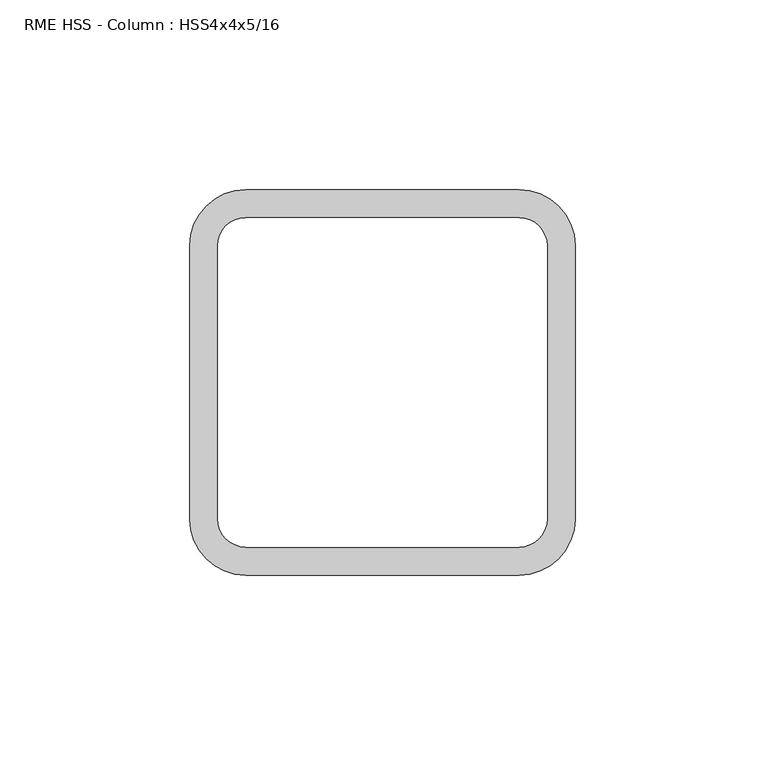
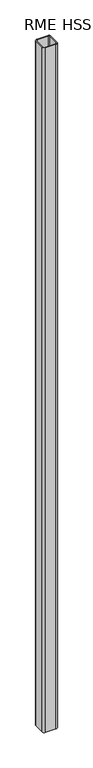
"""IFC4 building model written with IfcOpenShell, lengths in millimetres: column geometry, RME HSS - Column : HSS4x4x5/16."""

from ifc_helpers import new_model, si_unit, point, frame, frame_2d, origin, place, context, project, spatial, polyline, circle_curve, trimmed, segment, composite_curve, outline, extrude, source, transform, mapped, element, save


def rme_hss_column_hss4x4x5_16_e47b2026(model_context):
    return source(origin(), model_context, "Body", "SweptSolid", [
        extrude(outline(composite_curve([segment(trimmed(circle_curve(frame_2d((36.0172, 36.0172)), 14.7828), [point((36.0172, 50.8))], [point((50.8, 36.0172))], False, "CARTESIAN"), True, "CONTINUOUS"), segment(polyline([(50.8, 36.0172), (50.8, -36.0172)]), True, "CONTINUOUS"), segment(trimmed(circle_curve(frame_2d((36.0172, -36.0172)), 14.7828), [point((50.8, -36.0172))], [point((36.0172, -50.8))], False, "CARTESIAN"), True, "CONTINUOUS"), segment(polyline([(36.0172, -50.8), (-36.0172, -50.8)]), True, "CONTINUOUS"), segment(trimmed(circle_curve(frame_2d((-36.0172, -36.0172)), 14.7828), [point((-36.0172, -50.8))], [point((-50.8, -36.0172))], False, "CARTESIAN"), True, "CONTINUOUS"), segment(polyline([(-50.8, -36.0172), (-50.8, 36.0172)]), True, "CONTINUOUS"), segment(trimmed(circle_curve(frame_2d((-36.0172, 36.0172)), 14.7828), [point((-50.8, 36.0172))], [point((-36.0172, 50.8))], False, "CARTESIAN"), True, "CONTINUOUS"), segment(polyline([(-36.0172, 50.8), (36.0172, 50.8)]), True, "CONTINUOUS")], self_intersect=False), holes=[composite_curve([segment(polyline([(36.0172, 43.4086), (-36.0172, 43.4086)]), True, "CONTINUOUS"), segment(trimmed(circle_curve(frame_2d((-36.0172, 36.0172)), 7.3914), [point((-36.0172, 43.4086))], [point((-43.4086, 36.0172))], True, "CARTESIAN"), True, "CONTINUOUS"), segment(polyline([(-43.4086, 36.0172), (-43.4086, -36.0172)]), True, "CONTINUOUS"), segment(trimmed(circle_curve(frame_2d((-36.0172, -36.0172)), 7.3914), [point((-43.4086, -36.0172))], [point((-36.0172, -43.4086))], True, "CARTESIAN"), True, "CONTINUOUS"), segment(polyline([(-36.0172, -43.4086), (36.0172, -43.4086)]), True, "CONTINUOUS"), segment(trimmed(circle_curve(frame_2d((36.0172, -36.0172)), 7.3914), [point((36.0172, -43.4086))], [point((43.4086, -36.0172))], True, "CARTESIAN"), True, "CONTINUOUS"), segment(polyline([(43.4086, -36.0172), (43.4086, 36.0172)]), True, "CONTINUOUS"), segment(trimmed(circle_curve(frame_2d((36.0172, 36.0172)), 7.3914), [point((43.4086, 36.0172))], [point((36.0172, 43.4086))], True, "CARTESIAN"), True, "CONTINUOUS")], self_intersect=False)]), frame((0.0, 0.0, -203.2), z_axis=(0.0, 0.0, 1.0), x_axis=(1.0, 0.0, 0.0)), (0.0, 0.0, 1.0), 4902.2),
    ])


if __name__ == "__main__":
    model = new_model("IFC4")
    model_context = context("Model", 3, world=origin())
    ifc_project = project(units=[si_unit("LENGTHUNIT", "METRE", prefix="MILLI")], contexts=[model_context])
    site = spatial("IfcSite", under=ifc_project)
    building = spatial("IfcBuilding", under=site)
    placement = place(None, origin())
    rme_hss_column_hss4x4x5_16_shape = rme_hss_column_hss4x4x5_16_e47b2026(model_context)
    element("IfcColumn", 1, ObjectType="RME HSS - Column : HSS4x4x5/16", at=placement, inside=building, context=model_context, shape_type="MappedRepresentation", body=[
        mapped(rme_hss_column_hss4x4x5_16_shape, transform((0.0, 0.0, 0.0), x_axis=(1.0, 0.0, 0.0), y_axis=(0.0, 1.0, 0.0), z_axis=(0.0, 0.0, 1.0))),
    ])
    save(model, "model.ifc")

# Revit data of these elements
# Type "RME HSS - Column : HSS4x4x5/16"
#   Nominal Size = ""
#   Base Plate Type [instance default] = ""
#   Assembly Code = "B10"
#   Shape = "Square"
#   W = 14.8
#   Ht = 0' - 4"
#   b = 0' - 4"
#   kr = 0' - 0.582"
#   t = 0' - 0.291"
#   A = 0.0284722 SF
#   Structural Material [instance default] = Metal - Steel - ASTM A500 - Grade B - Rectangular and Square
# Element 1 (IfcColumn, "RME HSS - Column : HSS4x4x5/16")
#   Materials on its faces: "Metal - Steel - ASTM A500 - Grade B - Rectangular and Square"
# Materials
#   "Metal - Steel - ASTM A500 - Grade B - Rectangular and Square": class "Metal", colour RGB 255 128 0, transparency 0
